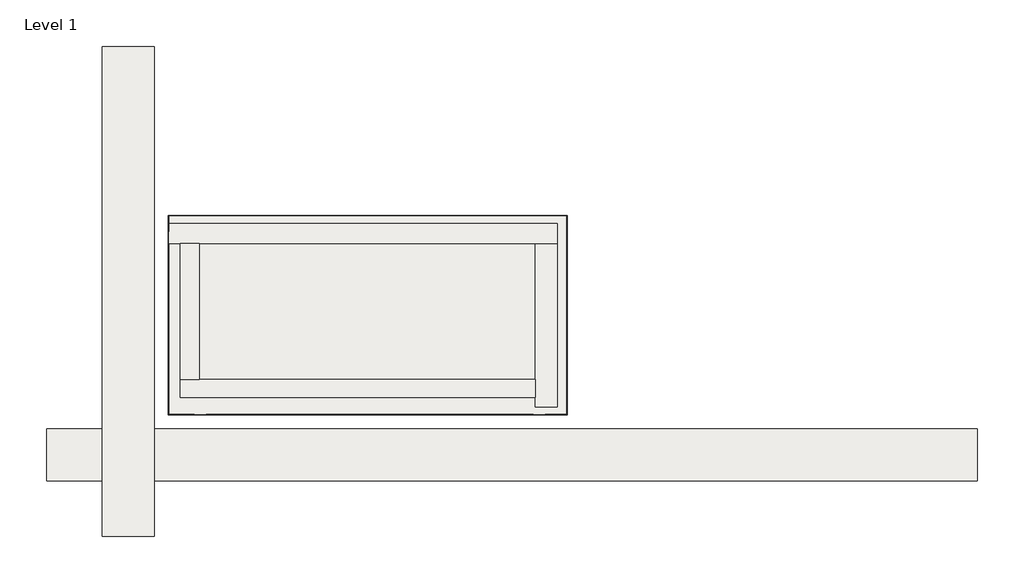
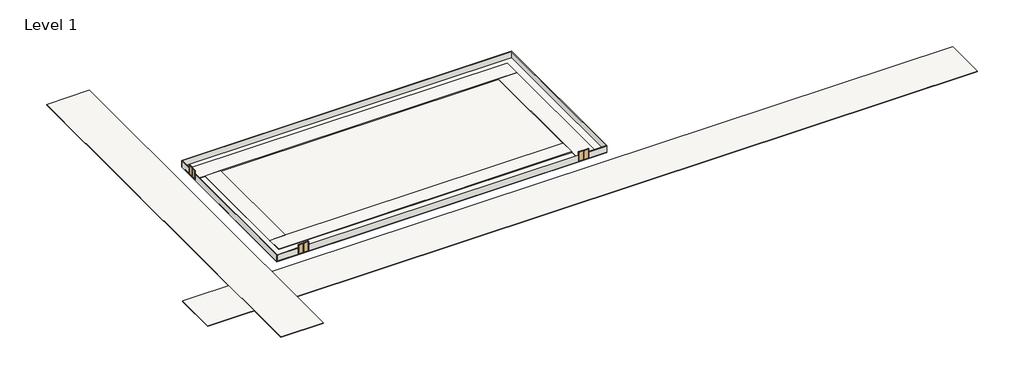
# One storey: 7 slabs, 4 walls, 3 doors.
"""IFC4 building model written with IfcOpenShell, lengths in millimetres."""

import ifcopenshell
import ifcopenshell.guid

model = None  # the IFC model being written
_history = None  # IfcOwnerHistory: only IFC2X3 demands one
_inside = {}  # id of a spatial element -> (the spatial element, [elements in it])
_under = {}  # id of a project, library or spatial element -> (it, [spatial elements below it])
_declared = {}  # id of a project -> (the project, [libraries it declares])
_typed = {}  # id of a type object -> (the type object, [elements of that type])
_made_of = {}  # id of a material, layer set ... -> (it, [elements and type objects made of it])


def new_model(schema):
    """Start an empty IFC model of exactly this schema.

    Asked for "IFC4X3", IfcOpenShell would pick the latest addendum, in which some entities
    have other attributes; the version numbers below select the first issue.
    IFC2X3 requires an IfcOwnerHistory on every rooted entity: one is made here for all.
    """
    global model, _history
    if schema == "IFC4X3":
        model = ifcopenshell.file(schema_version=(4, 3, 0, 0))
    else:
        model = ifcopenshell.file(schema=schema)
    _inside.clear()
    _under.clear()
    _declared.clear()
    _typed.clear()
    _made_of.clear()
    _history = None
    if model.schema == "IFC2X3":
        org = make("IfcOrganization", Name="unknown")
        user = make(
            "IfcPersonAndOrganization",
            ThePerson=make("IfcPerson", FamilyName="unknown"),
            TheOrganization=org,
        )
        app = make(
            "IfcApplication",
            ApplicationDeveloper=org,
            Version="unknown",
            ApplicationFullName="unknown",
            ApplicationIdentifier="unknown",
        )
        _history = make(
            "IfcOwnerHistory",
            OwningUser=user,
            OwningApplication=app,
            ChangeAction="ADDED",
            CreationDate=0,
        )
    return model


def make(cls, **values):
    """One entity of the class cls with the attributes given. An attribute that is None is left unset."""
    return model.create_entity(
        cls, **{name: value for name, value in values.items() if value is not None}
    )


def rooted(cls, **values):
    """An entity with a GlobalId (a new one), such as an element, a storey or a relation."""
    return make(cls, GlobalId=ifcopenshell.guid.new(), OwnerHistory=_history, **values)


def si_unit(unit_type, name, prefix=None):
    """IfcSIUnit, for example si_unit("LENGTHUNIT", "METRE", prefix="MILLI")."""
    return make("IfcSIUnit", UnitType=unit_type, Prefix=prefix, Name=name)


def assignment(units):
    """IfcUnitAssignment: the units of a project."""
    return None if units is None else make("IfcUnitAssignment", Units=units)


def point(xyz):
    """IfcCartesianPoint."""
    return None if xyz is None else make("IfcCartesianPoint", Coordinates=xyz)


def direction(xyz):
    """IfcDirection."""
    return None if xyz is None else make("IfcDirection", DirectionRatios=xyz)


def frame(location, z_axis=None, x_axis=None):
    """IfcAxis2Placement3D, a coordinate frame: its origin and axes. An axis left out is left unset."""
    return make(
        "IfcAxis2Placement3D",
        Location=point(location),
        Axis=direction(z_axis),
        RefDirection=direction(x_axis),
    )


def origin():
    """The frame at (0, 0, 0) with its axes left unset."""
    return frame((0.0, 0.0, 0.0))


def place(relative_to, where):
    """IfcLocalPlacement: puts the frame where relative to a parent placement (None: the world)."""
    return make(
        "IfcLocalPlacement", PlacementRelTo=relative_to, RelativePlacement=where
    )


def context(
    kind, dimensions, precision=None, world=None, true_north=None, identifier=None
):
    """IfcGeometricRepresentationContext, for example the 3D "Model" context."""
    return make(
        "IfcGeometricRepresentationContext",
        ContextIdentifier=identifier,
        ContextType=kind,
        CoordinateSpaceDimension=dimensions,
        Precision=precision,
        WorldCoordinateSystem=world,
        TrueNorth=true_north,
    )


def project(units=None, contexts=None):
    """IfcProject with its units and contexts."""
    return rooted(
        "IfcProject",
        Name="project",
        RepresentationContexts=contexts,
        UnitsInContext=assignment(units),
    )


def spatial(cls, under=None, at=None, **own):
    """A site, building, storey or space (cls), placed at a placement, below another one or the project."""
    s = rooted(cls, ObjectPlacement=at, **own)
    if under is not None:
        _under.setdefault(under.id(), (under, []))[1].append(s)
    return s


def polyline(points):
    """IfcPolyline through the points."""
    return make("IfcPolyline", Points=[point(p) for p in points])


def outline(outer, holes=None, kind="AREA"):
    """IfcArbitraryClosedProfileDef: a profile drawn as a closed curve; with holes, ...WithVoids."""
    if holes is None:
        return make("IfcArbitraryClosedProfileDef", ProfileType=kind, OuterCurve=outer)
    return make(
        "IfcArbitraryProfileDefWithVoids",
        ProfileType=kind,
        OuterCurve=outer,
        InnerCurves=holes,
    )


def extrude(swept, where, along, depth):
    """IfcExtrudedAreaSolid: the profile swept, set in the frame where, extruded along a direction by depth."""
    return make(
        "IfcExtrudedAreaSolid",
        SweptArea=swept,
        Position=where,
        ExtrudedDirection=direction(along),
        Depth=depth,
    )


def faces_of(points, faces, orient=None, outer=None):
    """IfcFace entities. A face is a list of loops; a loop is a list of indices into points, from 0.

    orient and outer hold one flag for each loop. By default every Orientation is true, the
    first loop of a face is its IfcFaceOuterBound and the others are IfcFaceBound.
    """
    made = []
    for i, loops in enumerate(faces):
        bounds = []
        for j, loop in enumerate(loops):
            is_outer = j == 0 if outer is None else outer[i][j]
            bounds.append(
                make(
                    "IfcFaceOuterBound" if is_outer else "IfcFaceBound",
                    Bound=make("IfcPolyLoop", Polygon=[points[k] for k in loop]),
                    Orientation=True if orient is None else orient[i][j],
                )
            )
        made.append(make("IfcFace", Bounds=bounds))
    return made


def faceted_brep(points, faces, orient=None, outer=None, voids=None):
    """IfcFacetedBrep: a solid bounded by flat faces; with voids (closed shells), ...WithVoids."""
    shared = [point(p) for p in points]
    hull = make("IfcClosedShell", CfsFaces=faces_of(shared, faces, orient, outer))
    if voids is None:
        return make("IfcFacetedBrep", Outer=hull)
    return make(
        "IfcFacetedBrepWithVoids",
        Outer=hull,
        Voids=[
            make(cls, CfsFaces=faces_of(shared, fs, o, b)) for cls, fs, o, b in voids
        ],
    )


def shape(context_of_items, identifier, shape_type, items):
    """IfcShapeRepresentation: the items that make up one representation, for example the "Body"."""
    return make(
        "IfcShapeRepresentation",
        ContextOfItems=context_of_items,
        RepresentationIdentifier=identifier,
        RepresentationType=shape_type,
        Items=items,
    )


def source(mapping_origin, context_of_items, identifier, shape_type, items):
    """IfcRepresentationMap: a shape defined once, which mapped items show again and again."""
    return make(
        "IfcRepresentationMap",
        MappingOrigin=mapping_origin,
        MappedRepresentation=shape(context_of_items, identifier, shape_type, items),
    )


def transform(
    local_origin,
    x_axis=None,
    y_axis=None,
    z_axis=None,
    scale=None,
    scale2=None,
    scale3=None,
    uniform=True,
):
    """IfcCartesianTransformationOperator3D, or its non-uniform kind. x_axis, y_axis, z_axis: its Axis1, 2, 3."""
    if uniform:
        return make(
            "IfcCartesianTransformationOperator3D",
            Axis1=direction(x_axis),
            Axis2=direction(y_axis),
            LocalOrigin=point(local_origin),
            Scale=scale,
            Axis3=direction(z_axis),
        )
    return make(
        "IfcCartesianTransformationOperator3DnonUniform",
        Axis1=direction(x_axis),
        Axis2=direction(y_axis),
        LocalOrigin=point(local_origin),
        Scale=scale,
        Axis3=direction(z_axis),
        Scale2=scale2,
        Scale3=scale3,
    )


def mapped(mapping_source, mapping_target):
    """IfcMappedItem: shows the shape of a source again, moved by a transform."""
    return make(
        "IfcMappedItem", MappingSource=mapping_source, MappingTarget=mapping_target
    )


def made_of(thing, what):
    """Note that an element or type object is made of a material, layer set ...; save() writes the relation."""
    if what is not None:
        _made_of.setdefault(what.id(), (what, []))[1].append(thing)
    return thing


def element(
    cls,
    number,
    at=None,
    inside=None,
    cuts=None,
    type_object=None,
    material=None,
    context=None,
    identifier="Body",
    shape_type=None,
    held_by="IfcProductDefinitionShape",
    body=None,
    shapes=None,
    **own,
):
    """One element of the class cls, such as IfcWall. Its Tag is "e" and its number.

    at: its placement. inside: the storey or other place that contains it. cuts: it is an
    opening in that element (IfcRelVoidsElement). A single representation is given by context,
    identifier, shape_type and body (its items); several are given by shapes. held_by: the class
    of the entity that holds the representations. save() writes the other relations.
    """
    e = rooted(cls, Tag="e%d" % number, ObjectPlacement=at, **own)
    if body is not None:
        shapes = [shape(context, identifier, shape_type, body)]
    if shapes is not None:
        e.Representation = make(held_by, Representations=shapes)
    if inside is not None:
        _inside.setdefault(inside.id(), (inside, []))[1].append(e)
    if cuts is not None:
        rooted(
            "IfcRelVoidsElement", RelatingBuildingElement=cuts, RelatedOpeningElement=e
        )
    if type_object is not None:
        _typed.setdefault(type_object.id(), (type_object, []))[1].append(e)
    return made_of(e, material)


def aggregate(whole, parts):
    """IfcRelAggregates: a whole, such as a stair, and the parts it consists of."""
    return rooted("IfcRelAggregates", RelatingObject=whole, RelatedObjects=parts)


def save(model, path):
    """Write the relations noted so far, then the file.

    IfcRelAggregates (storeys below a building ...), IfcRelContainedInSpatialStructure (elements
    in a storey), IfcRelDefinesByType, IfcRelAssociatesMaterial and IfcRelDeclares: one each for
    every whole, place, type object, material and project.
    """
    for whole, parts in _under.values():
        aggregate(whole, parts)
    for where, things in _inside.values():
        rooted(
            "IfcRelContainedInSpatialStructure",
            RelatedElements=things,
            RelatingStructure=where,
        )
    for kind, things in _typed.values():
        rooted("IfcRelDefinesByType", RelatedObjects=things, RelatingType=kind)
    for what, things in _made_of.values():
        rooted("IfcRelAssociatesMaterial", RelatedObjects=things, RelatingMaterial=what)
    for by, libraries in _declared.values():
        rooted("IfcRelDeclares", RelatingContext=by, RelatedDefinitions=libraries)
    model.write(path)


def m_door_double_glass_6000x6000_a7e1d600(model_context):
    return source(origin(), model_context, "Body", "SweptSolid", [
        extrude(outline(polyline([(6000.0, -3000.0), (0.0, -3000.0), (0.0, 0.0), (6000.0, 0.0), (6000.0, -3000.0)]), holes=[polyline([(5900.0, -2900.0), (5900.0, -100.0), (100.0, -100.0), (100.0, -2900.0), (5900.0, -2900.0)])]), frame((0.0, 52.38125, 0.0), z_axis=(0.0, 1.0, 0.0), x_axis=(0.0, 0.0, 1.0)), (0.0, 0.0, 1.0), 50.0),
        extrude(outline(polyline([(6000.0, 3000.0), (6000.0, 0.0), (0.0, 0.0), (0.0, 3000.0), (6000.0, 3000.0)]), holes=[polyline([(5900.0, 2900.0), (100.0, 2900.0), (100.0, 100.0), (5900.0, 100.0), (5900.0, 2900.0)])]), frame((0.0, 52.38125, 0.0), z_axis=(0.0, 1.0, 0.0), x_axis=(0.0, 0.0, 1.0)), (0.0, 0.0, 1.0), 50.0),
        extrude(outline(polyline([(100.0, 80.55625), (2900.0, 80.55625), (2900.0, 74.20625), (100.0, 74.20625), (100.0, 80.55625)])), frame((0.0, 0.0, 100.0), z_axis=(0.0, 0.0, 1.0), x_axis=(1.0, 0.0, 0.0)), (0.0, 0.0, 1.0), 5800.0),
        extrude(outline(polyline([(-2900.0, 80.55625), (-100.0, 80.55625), (-100.0, 74.20625), (-2900.0, 74.20625), (-2900.0, 80.55625)])), frame((0.0, 0.0, 100.0), z_axis=(0.0, 0.0, 1.0), x_axis=(1.0, 0.0, 0.0)), (0.0, 0.0, 1.0), 5800.0),
        extrude(outline(polyline([(0.0, 3080.0), (6080.0, 3080.0), (6080.0, -3080.0), (0.0, -3080.0), (0.0, -3000.0), (6000.0, -3000.0), (6000.0, 3000.0), (0.0, 3000.0), (0.0, 3080.0)])), frame((0.0, 102.38125, 0.0), z_axis=(0.0, 1.0, 0.0), x_axis=(0.0, 0.0, 1.0)), (0.0, 0.0, 1.0), 25.0),
        extrude(outline(polyline([(0.0, 3080.0), (6080.0, 3080.0), (6080.0, -3080.0), (0.0, -3080.0), (0.0, -3000.0), (6000.0, -3000.0), (6000.0, 3000.0), (0.0, 3000.0), (0.0, 3080.0)])), frame((0.0, -122.61875, 0.0), z_axis=(0.0, 1.0, 0.0), x_axis=(0.0, 0.0, 1.0)), (0.0, 0.0, 1.0), 25.0),
    ])


model = new_model("IFC4")

# Units and contexts
model_context = context("Model", 3, world=origin())
ifc_project = project(units=[si_unit("LENGTHUNIT", "METRE", prefix="MILLI")], contexts=[model_context])

# Site, building, storey
site = spatial("IfcSite", under=ifc_project)
building = spatial("IfcBuilding", under=site)
storey = spatial("IfcBuildingStorey", under=building, Name="Level 1", Elevation=0.0)

# Doors
placement = place(None, origin())
m_door_double_glass_6000x6000_shape = m_door_double_glass_6000x6000_a7e1d600(model_context)
element("IfcDoor", 1, ObjectType="M_Door-Double-Glass : 6000x6000", at=placement, inside=storey, context=model_context, shape_type="MappedRepresentation", body=[
    mapped(m_door_double_glass_6000x6000_shape, transform((-168891.0003458, -94498.6580522, 0.0), x_axis=(-1.0, 0.0, 0.0), y_axis=(0.0, -1.0, 0.0), z_axis=(0.0, 0.0, 1.0))),
])
element("IfcDoor", 2, ObjectType="M_Door-Double-Glass : 6000x6000", at=placement, inside=storey, context=model_context, shape_type="MappedRepresentation", body=[
    mapped(m_door_double_glass_6000x6000_shape, transform((-184888.6190958, -5501.0393022, 0.0), x_axis=(0.0, 1.0, 0.0), y_axis=(-1.0, 0.0, 0.0), z_axis=(0.0, 0.0, 1.0))),
])
element("IfcDoor", 3, ObjectType="M_Door-Double-Glass : 6000x6000", at=placement, inside=storey, context=model_context, shape_type="MappedRepresentation", body=[
    mapped(m_door_double_glass_6000x6000_shape, transform((1108.9996542, -94498.6580522, 0.0), x_axis=(-1.0, 0.0, 0.0), y_axis=(0.0, -1.0, 0.0), z_axis=(0.0, 0.0, 1.0))),
])

# Slabs
element("IfcSlab", 4, ObjectType="Generic Floor - 400mm", at=placement, inside=storey, context=model_context, shape_type="SweptSolid", body=[
    extrude(outline(polyline([(-184891.0003458, 5498.9606978), (15108.9996542, 5498.9606978), (15108.9996542, -94501.0393022), (-184891.0003458, -94501.0393022), (-184891.0003458, 5498.9606978)])), frame((0.0, 0.0, -400.0), z_axis=(0.0, 0.0, 1.0), x_axis=(1.0, 0.0, 0.0)), (0.0, 0.0, 1.0), 400.0),
])
element("IfcSlab", 5, ObjectType="Generic Floor - 400mm", at=placement, inside=storey, context=model_context, shape_type="SweptSolid", body=[
    extrude(outline(polyline([(-217965.448184, 90378.983425), (-191965.448184, 90378.983425), (-191965.448184, -155621.016575), (-217965.448184, -155621.016575), (-217965.448184, 90378.983425)])), frame((0.0, 0.0, -400.0), z_axis=(0.0, 0.0, 1.0), x_axis=(1.0, 0.0, 0.0)), (0.0, 0.0, 1.0), 400.0),
])
element("IfcSlab", 6, ObjectType="Generic Floor - 400mm", at=placement, inside=storey, context=model_context, shape_type="SweptSolid", body=[
    extrude(outline(polyline([(220989.0223815, -127575.4871405), (-246010.9776185, -127575.4871405), (-246010.9776185, -101575.4871405), (220989.0223815, -101575.4871405), (220989.0223815, -127575.4871405)])), frame((0.0, 0.0, -400.0), z_axis=(0.0, 0.0, 1.0), x_axis=(1.0, 0.0, 0.0)), (0.0, 0.0, 1.0), 400.0),
])
element("IfcSlab", 7, ObjectType="Generic Floor - 400mm", at=placement, inside=storey, context=model_context, shape_type="Brep", body=[
    faceted_brep([(-184991.0003458, 1478.3217568, 100.0), (10108.9996542, 1478.3217568, 100.0), (10108.9996542, -8501.0393022, 100.0), (-891.0003458, -8501.0393022, 100.0), (-169528.784266, -8501.0393022, 100.0), (-178891.0003458, -8501.0393022, 100.0), (-184991.0003458, -8501.0393022, 100.0), (-184991.0003458, 1478.3217568, 500.0), (-184991.0003458, -8501.0393022, 500.0), (-178891.0003458, -8501.0393022, 500.0), (-169528.784266, -8501.0393022, 500.0), (-891.0003458, -8501.0393022, 500.0), (10108.9996542, -8501.0393022, 500.0), (10108.9996542, 1478.3217568, 500.0)], [[[0, 1, 2, 3, 4, 5, 6]], [[7, 8, 9, 10, 11, 12, 13]], [[1, 0, 7, 13]], [[2, 1, 13, 12]], [[6, 5, 4, 3, 2, 12, 11, 10, 9, 8]], [[0, 6, 8, 7]]]),
])
element("IfcSlab", 8, ObjectType="Generic Floor - 400mm", at=placement, inside=storey, context=model_context, shape_type="Brep", body=[
    faceted_brep([(-891.0003458, -8501.0393022, 100.0), (10108.9996542, -8501.0393022, 100.0), (10108.9996542, -90501.0393022, 100.0), (-891.0003458, -90501.0393022, 100.0), (-891.0003458, -85758.4340045, 100.0), (-891.0003458, -76758.4340045, 100.0), (-891.0003458, -8501.0393022, 500.0), (-891.0003458, -76758.4340045, 500.0), (-891.0003458, -85758.4340045, 500.0), (-891.0003458, -90501.0393022, 500.0), (10108.9996542, -90501.0393022, 500.0), (10108.9996542, -8501.0393022, 500.0)], [[[0, 1, 2, 3, 4, 5]], [[6, 7, 8, 9, 10, 11]], [[1, 0, 6, 11]], [[2, 1, 11, 10]], [[3, 2, 10, 9]], [[0, 5, 4, 3, 9, 8, 7, 6]]]),
])
element("IfcSlab", 9, ObjectType="Generic Floor - 400mm", at=placement, inside=storey, context=model_context, shape_type="Brep", body=[
    faceted_brep([(-178891.0003458, -76758.4340045, 100.0), (-169528.784266, -76758.4340045, 100.0), (-891.0003458, -76758.4340045, 100.0), (-891.0003458, -85758.4340045, 100.0), (-178891.0003458, -85758.4340045, 100.0), (-178891.0003458, -76758.4340045, 500.0), (-178891.0003458, -85758.4340045, 500.0), (-891.0003458, -85758.4340045, 500.0), (-891.0003458, -76758.4340045, 500.0), (-169528.784266, -76758.4340045, 500.0)], [[[0, 1, 2, 3, 4]], [[5, 6, 7, 8, 9]], [[2, 1, 0, 5, 9, 8]], [[3, 2, 8, 7]], [[4, 3, 7, 6]], [[0, 4, 6, 5]]]),
])
element("IfcSlab", 10, ObjectType="Generic Floor - 400mm", at=placement, inside=storey, context=model_context, shape_type="SweptSolid", body=[
    extrude(outline(polyline([(-169528.784266, -76758.4340045), (-178891.0003458, -76758.4340045), (-178891.0003458, -8501.0393022), (-169528.784266, -8501.0393022), (-169528.784266, -76758.4340045)])), frame((0.0, 0.0, 100.0), z_axis=(0.0, 0.0, 1.0), x_axis=(1.0, 0.0, 0.0)), (0.0, 0.0, 1.0), 400.0),
])

# Walls
element("IfcWall", 11, ObjectType="Generic - 200mm", at=placement, inside=storey, context=model_context, shape_type="Brep", body=[
    faceted_brep([(-184991.0003458, -94601.0393022, 0.0), (-184991.0003458, -94601.0393022, 4000.0), (-184991.0003458, -8501.0393022, 4000.0), (-184991.0003458, -8501.0393022, 0.0), (-184791.0003458, -94601.0393022, 4000.0), (-184791.0003458, -94601.0393022, 0.0), (-184791.0003458, -94401.0393022, 0.0), (-184791.0003458, -8501.0393022, 0.0), (-184791.0003458, -8501.0393022, 4000.0), (-184791.0003458, -94401.0393022, 4000.0)], [[[0, 1, 2, 3]], [[4, 5, 6, 7, 8, 9]], [[5, 0, 3, 7, 6]], [[1, 4, 9, 8, 2]], [[1, 0, 5, 4]], [[3, 2, 8, 7]]]),
    faceted_brep([(-184991.0003458, 5398.9606978, 4000.0), (-184991.0003458, 5398.9606978, 0.0), (-184991.0003458, -2501.0393022, 0.0), (-184991.0003458, -2501.0393022, 4000.0), (-184791.0003458, 5398.9606978, 0.0), (-184791.0003458, 5398.9606978, 4000.0), (-184791.0003458, -2501.0393022, 4000.0), (-184791.0003458, -2501.0393022, 0.0)], [[[0, 1, 2, 3]], [[4, 5, 6, 7]], [[1, 4, 7, 2]], [[5, 0, 3, 6]], [[1, 0, 5, 4]], [[3, 2, 7, 6]]]),
])
element("IfcWall", 12, ObjectType="Generic - 200mm", at=placement, inside=storey, context=model_context, shape_type="Brep", body=[
    faceted_brep([(15208.9996542, -94601.0393022, 0.0), (15208.9996542, -94601.0393022, 4000.0), (4108.9996542, -94601.0393022, 4000.0), (4108.9996542, -94601.0393022, 0.0), (15208.9996542, -94401.0393022, 4000.0), (15208.9996542, -94401.0393022, 0.0), (15008.9996542, -94401.0393022, 0.0), (4108.9996542, -94401.0393022, 0.0), (4108.9996542, -94401.0393022, 4000.0), (15008.9996542, -94401.0393022, 4000.0)], [[[0, 1, 2, 3]], [[4, 5, 6, 7, 8, 9]], [[5, 0, 3, 7, 6]], [[1, 4, 9, 8, 2]], [[1, 0, 5, 4]], [[3, 2, 8, 7]]]),
    faceted_brep([(-184791.0003458, -94601.0393022, 4000.0), (-184791.0003458, -94601.0393022, 0.0), (-171891.0003458, -94601.0393022, 0.0), (-171891.0003458, -94601.0393022, 4000.0), (-184791.0003458, -94401.0393022, 0.0), (-184791.0003458, -94401.0393022, 4000.0), (-171891.0003458, -94401.0393022, 4000.0), (-171891.0003458, -94401.0393022, 0.0)], [[[0, 1, 2, 3]], [[4, 5, 6, 7]], [[1, 4, 7, 2]], [[5, 0, 3, 6]], [[1, 0, 5, 4]], [[3, 2, 7, 6]]]),
    faceted_brep([(-165891.0003458, -94601.0393022, 4000.0), (-165891.0003458, -94601.0393022, 0.0), (-1891.0003458, -94601.0393022, 0.0), (-1891.0003458, -94601.0393022, 4000.0), (-165891.0003458, -94401.0393022, 0.0), (-165891.0003458, -94401.0393022, 4000.0), (-1891.0003458, -94401.0393022, 4000.0), (-1891.0003458, -94401.0393022, 0.0)], [[[0, 1, 2, 3]], [[4, 5, 6, 7]], [[1, 4, 7, 2]], [[5, 0, 3, 6]], [[1, 0, 5, 4]], [[3, 2, 7, 6]]]),
])
element("IfcWall", 13, ObjectType="Generic - 200mm", at=placement, inside=storey, context=model_context, shape_type="Brep", body=[
    faceted_brep([(15208.9996542, -94401.0393022, 0.0), (15208.9996542, 5598.9606978, 0.0), (15208.9996542, 5598.9606978, 4000.0), (15208.9996542, -94401.0393022, 4000.0), (15008.9996542, -94401.0393022, 0.0), (15008.9996542, -94401.0393022, 4000.0), (15008.9996542, 5398.9606978, 4000.0), (15008.9996542, 5598.9606978, 4000.0), (15008.9996542, 5598.9606978, 0.0), (15008.9996542, 5398.9606978, 0.0)], [[[0, 1, 2, 3]], [[4, 5, 6, 7, 8, 9]], [[1, 0, 4, 9, 8]], [[3, 2, 7, 6, 5]], [[2, 1, 8, 7]], [[0, 3, 5, 4]]]),
])
element("IfcWall", 14, ObjectType="Generic - 200mm", at=placement, inside=storey, context=model_context, shape_type="Brep", body=[
    faceted_brep([(15008.9996542, 5598.9606978, 0.0), (-184991.0003458, 5598.9606978, 0.0), (-184991.0003458, 5598.9606978, 4000.0), (15008.9996542, 5598.9606978, 4000.0), (15008.9996542, 5398.9606978, 0.0), (15008.9996542, 5398.9606978, 4000.0), (-184791.0003458, 5398.9606978, 4000.0), (-184991.0003458, 5398.9606978, 4000.0), (-184991.0003458, 5398.9606978, 0.0), (-184791.0003458, 5398.9606978, 0.0)], [[[0, 1, 2, 3]], [[4, 5, 6, 7, 8, 9]], [[1, 0, 4, 9, 8]], [[3, 2, 7, 6, 5]], [[2, 1, 8, 7]], [[0, 3, 5, 4]]]),
])

save(model, "model.ifc")

# Revit data of these elements
# Project information
#   Project Issue Date = "Issue Date"
#   Project Status = "Project  Status"
#   Client Name = "Owner"
#   Project Address = "## Street\nCity, State  Zip"
#   Project Name = "Project Name"
#   Project Number = "0001"
#   SR Document GUID = "9cbb99a4-4d3b-4e58-9c09-d180e02345c8"
# Type "M_Door-Double-Glass : 6000x6000"
#   Type Mark = "22"
#   Construction Type Id = "opn-d45"
#   Assembly Code = "C1020"
#   Analytic Construction = "Wood frame, double glass door "
#   W = 3000 mm
#   Thickness = 50 mm
#   Thermal Resistance (R) = 0.31964 (m²·K)/W
#   Swing Angle [instance default] = 90.00°
#   Heat Transfer Coefficient (U) = 3.12872 W/(m²·K)
#   Height = 6000 mm
#   Bottom Rail = 100 mm
#   Top Rail = 100 mm
#   Stiles = 100 mm
#   Trim Projection = 25 mm
#   Trim Width = 80 mm
#   Width = 6000 mm
#   Glazing = Glass
#   Panel Material = Wood - Birch - Solid Stained Light Low Gloss
#   Trim Material = Paint - Sienna
#   Visual Light Transmittance = 0
#   Solar Heat Gain Coefficient = 0
#   Function = (empty or 0)
#   Wall Closure = (empty or 0)
# Type "Generic Floor - 400mm"
#   Function = 0
#   Layers, outside or top first: 400 mm no material (function 1)
# Type "Generic - 200mm"
#   Layers, outside or top first: 200 mm no material (function 1)
# Elements 1, 2, 3 (IfcDoor, "M_Door-Double-Glass : 6000x6000")
#   Swing Angle = 90.00°
#   Phase Created = New Construction
#   Materials on its faces: "Wood - Birch - Solid Stained Light Low Gloss", "Paint - Sienna", "Glass"
# Elements 4, 5 (IfcSlab, "Generic Floor - 400mm")
#   built-in parameter 1001955 = 3.14159 (stored number, unit not read)
#   Height Offset From Level = 0 mm
#   Phase Created = New Construction
#   Materials on its faces: "Default Roof"
# Element 6 (IfcSlab, "Generic Floor - 400mm")
#   built-in parameter 1001955 = -1.5708 (stored number, unit not read)
#   Height Offset From Level = 0 mm
#   Phase Created = New Construction
#   Materials on its faces: "Default Roof"
# Elements 7, 8, 9 (IfcSlab, "Generic Floor - 400mm")
#   built-in parameter 1001955 = 3.14159 (stored number, unit not read)
#   Height Offset From Level = 500 mm
#   Phase Created = New Construction
#   Materials on its faces: "Default Roof"
# Element 10 (IfcSlab, "Generic Floor - 400mm")
#   Height Offset From Level = 500 mm
#   Phase Created = New Construction
#   Materials on its faces: "Default Roof"
# Elements 11, 12, 13, 14 (IfcWall, "Generic - 200mm")
#   Top Offset = 0 mm
#   Base Offset = 0 mm
#   Unconnected Height = 4000 mm
#   wall height = 4000 mm
#   Phase Created = New Construction
#   Base Constraint = Level 1
#   Materials on its faces: "Default Wall"
# Materials
#   "Glass": class "Glass", colour RGB 0 128 192, transparency 0.75, Description = "Soda Lime Glass", Cost = 0
#   "Wood - Birch - Solid Stained Light Low Gloss": class "Wood", colour RGB 210 159 95, transparency 0, Cost = 0
#   "Paint - Sienna": class "Miscellaneous", colour RGB 118 70 51, transparency 0, Cost = 0
#   "Default Roof": class "Miscellaneous", colour RGB 88 101 114, transparency 0, Cost = 0
#   "Default Wall": class "Miscellaneous", colour RGB 128 128 128, transparency 0, Cost = 0
